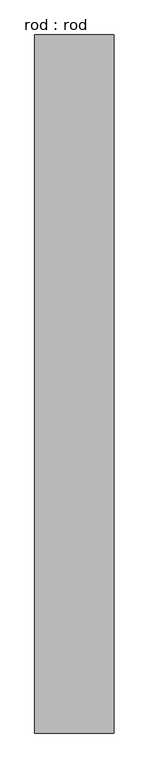
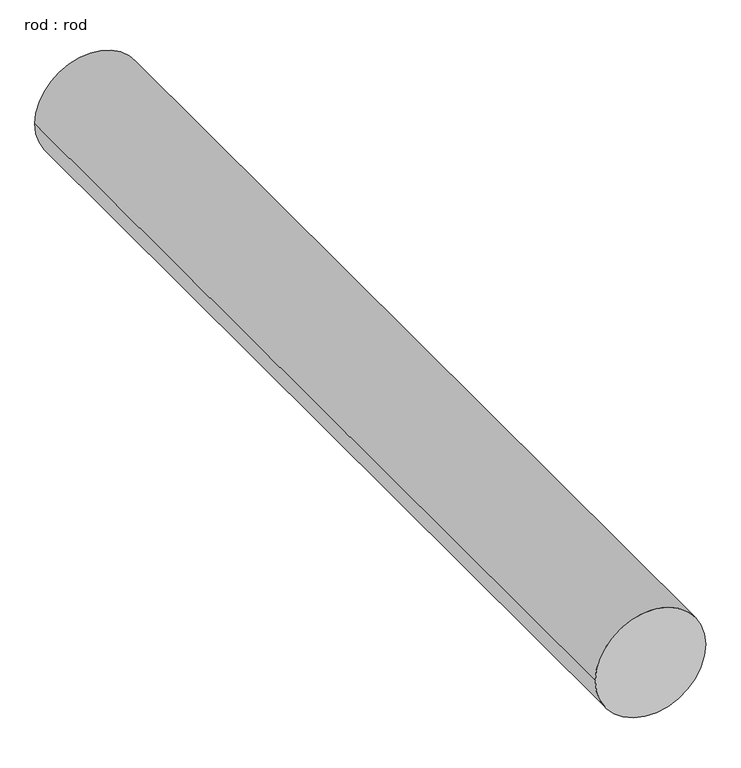
"""IFC4 building model written with IfcOpenShell, lengths in millimetres: proxy geometry, rod : rod."""

from ifc_helpers import new_model, si_unit, point, frame, frame_2d, origin, place, context, project, spatial, circle_curve, trimmed, segment, composite_curve, outline, extrude, source, transform, mapped, element, save


def rod_rod_335604b2(model_context):
    return source(origin(), model_context, "Body", "SweptSolid", [
        extrude(outline(composite_curve([segment(trimmed(circle_curve(frame_2d((0.0108462, 0.0)), 200.0), [point((0.0108462, 200.0))], [point((0.0108462, -200.0))], False, "CARTESIAN"), True, "CONTINUOUS"), segment(trimmed(circle_curve(frame_2d((0.0108462, 0.0)), 200.0), [point((0.0108462, -200.0))], [point((0.0108462, 200.0))], False, "CARTESIAN"), True, "CONTINUOUS")], self_intersect=False)), frame((0.0, 2332.7286153, 0.0), z_axis=(0.0, 1.0, 0.0), x_axis=(0.0, 0.0, 1.0)), (0.0, 0.0, 1.0), 3520.0),
    ])


if __name__ == "__main__":
    model = new_model("IFC4")
    model_context = context("Model", 3, world=origin())
    ifc_project = project(units=[si_unit("LENGTHUNIT", "METRE", prefix="MILLI")], contexts=[model_context])
    site = spatial("IfcSite", under=ifc_project)
    building = spatial("IfcBuilding", under=site)
    placement = place(None, origin())
    rod_rod_shape = rod_rod_335604b2(model_context)
    element("IfcBuildingElementProxy", 1, Name="rod : rod", ObjectType="rod : rod", at=placement, inside=building, context=model_context, shape_type="MappedRepresentation", body=[
        mapped(rod_rod_shape, transform((0.0, 0.0, 0.0), x_axis=(1.0, 0.0, 0.0), y_axis=(0.0, 1.0, 0.0), z_axis=(0.0, 0.0, 1.0))),
    ])
    save(model, "model.ifc")

# Revit data of these elements
# Type "rod : rod"
#   Default Elevation = 0
